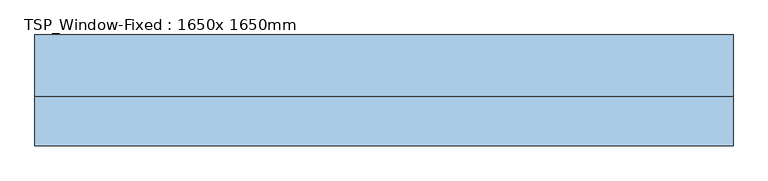
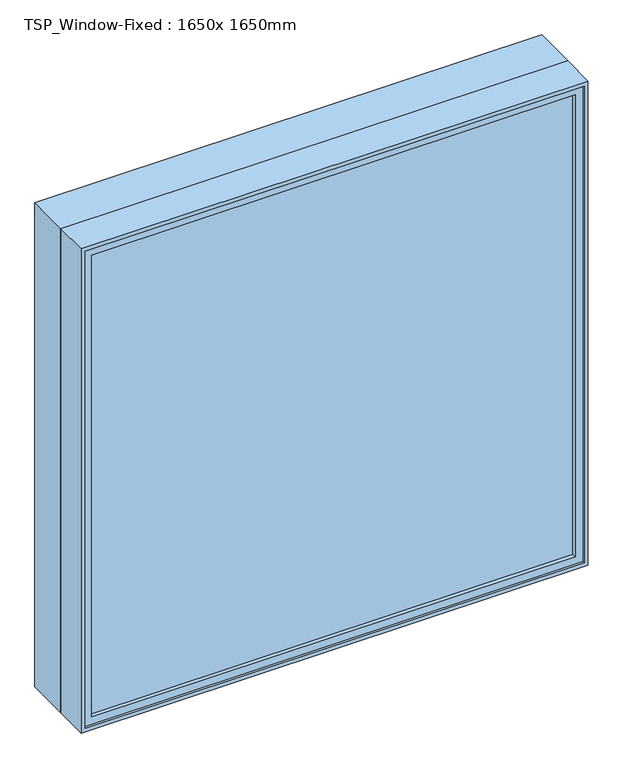
"""IFC4 building model written with IfcOpenShell, lengths in millimetres: window geometry, TSP_Window-Fixed : 1650x 1650mm."""

from ifc_helpers import new_model, si_unit, frame, origin, place, context, project, spatial, polyline, outline, extrude, faceted_brep, source, transform, mapped, element, save


def tsp_window_fixed_1650x_1650mm_face6f7b(model_context):
    return source(origin(), model_context, "Body", "SolidModel", [
        faceted_brep([(817.5, -24.75, 2550.0), (-817.5, -24.75, 2550.0), (-817.5, -139.05, 2550.0), (817.5, -139.05, 2550.0), (-817.5, -24.75, 900.0), (-817.5, -139.05, 900.0), (817.5, -24.75, 900.0), (817.5, -139.05, 900.0), (785.75, -24.75, 2518.25), (-785.75, -24.75, 2518.25), (-785.75, -24.75, 931.75), (785.75, -24.75, 931.75), (-804.8, -139.05, 2537.3), (804.8, -139.05, 2537.3), (804.8, -139.05, 912.7), (-804.8, -139.05, 912.7), (785.75, -88.25, 2518.25), (-785.75, -88.25, 2518.25), (-804.8, -88.25, 2537.3), (804.8, -88.25, 2537.3), (-785.75, -88.25, 931.75), (-804.8, -88.25, 912.7), (785.75, -88.25, 931.75), (804.8, -88.25, 912.7)], [[[0, 1, 2, 3]], [[1, 4, 5, 2]], [[4, 6, 7, 5]], [[1, 0, 6, 4], [8, 9, 10, 11]], [[6, 0, 3, 7]], [[3, 2, 5, 7], [12, 13, 14, 15]], [[16, 17, 9, 8]], [[13, 12, 18, 19]], [[17, 20, 10, 9]], [[12, 15, 21, 18]], [[20, 22, 11, 10]], [[15, 14, 23, 21]], [[22, 16, 8, 11]], [[19, 18, 21, 23], [17, 16, 22, 20]], [[14, 13, 19, 23]]]),
        extrude(outline(polyline([(2550.0, -817.5), (900.0, -817.5), (900.0, 817.5), (2550.0, 817.5), (2550.0, -817.5)]), holes=[polyline([(2537.3, 804.8), (912.7, 804.8), (912.7, -804.8), (2537.3, -804.8), (2537.3, 804.8)])]), frame((0.0, -24.75, 0.0), z_axis=(0.0, 1.0, 0.0), x_axis=(0.0, 0.0, 1.0)), (0.0, 0.0, 1.0), 144.75),
        extrude(outline(polyline([(912.7, -804.8), (912.7, 804.8), (2537.3, 804.8), (2537.3, -804.8), (912.7, -804.8)]), holes=[polyline([(938.1, 779.4), (938.1, -779.4), (2511.9, -779.4), (2511.9, 779.4), (938.1, 779.4)])]), frame((0.0, -132.7, 0.0), z_axis=(0.0, 1.0, 0.0), x_axis=(0.0, 0.0, 1.0)), (0.0, 0.0, 1.0), 44.45),
        extrude(outline(polyline([(779.4, -120.0), (-779.4, -120.0), (-779.4, -113.65), (779.4, -113.65), (779.4, -120.0)])), frame((0.0, 0.0, 938.1), z_axis=(0.0, 0.0, 1.0), x_axis=(1.0, 0.0, 0.0)), (0.0, 0.0, 1.0), 1573.8),
        extrude(outline(polyline([(-779.4, -100.95), (779.4, -100.95), (779.4, -107.3), (-779.4, -107.3), (-779.4, -100.95)])), frame((0.0, 0.0, 938.1), z_axis=(0.0, 0.0, 1.0), x_axis=(1.0, 0.0, 0.0)), (0.0, 0.0, 1.0), 1573.8),
    ])


if __name__ == "__main__":
    model = new_model("IFC4")
    model_context = context("Model", 3, world=origin())
    ifc_project = project(units=[si_unit("LENGTHUNIT", "METRE", prefix="MILLI")], contexts=[model_context])
    site = spatial("IfcSite", under=ifc_project)
    building = spatial("IfcBuilding", under=site)
    placement = place(None, origin())
    tsp_window_fixed_1650x_1650mm_shape = tsp_window_fixed_1650x_1650mm_face6f7b(model_context)
    element("IfcWindow", 1, ObjectType="TSP_Window-Fixed : 1650x 1650mm", at=placement, inside=building, context=model_context, shape_type="MappedRepresentation", body=[
        mapped(tsp_window_fixed_1650x_1650mm_shape, transform((0.0, 0.0, 0.0), x_axis=(1.0, 0.0, 0.0), y_axis=(0.0, 1.0, 0.0), z_axis=(0.0, 0.0, 1.0))),
    ])
    save(model, "model.ifc")

# Revit data of these elements
# Type "TSP_Window-Fixed : 1650x 1650mm"
#   Type Mark = "HS 2412 F154"
#   Fire Rating = "0.5h"
#   Assembly Code = "B2020100"
#   Analytic Construction = "Double glazing - domestic"
#   Window Inset [instance default] = 0 mm
#   Wall Thickness [instance default] = 150 mm
#   Visual Light Transmittance = 0.81
#   Thermal Resistance (R) = 0.319569 (m²·K)/W
#   Solar Heat Gain Coefficient = 0.76
#   Rough Width = 1650 mm
#   Rough Height = 1665 mm
#   Interior Wall Closure [instance default] = 54.75 mm
#   Height = 1650 mm
#   Heat Transfer Coefficient (U) = 3.12929 W/(m²·K)
#   Frame Extension [instance default] = 6.35 mm
#   Exterior Wall Closure [instance default] = 31.75 mm
#   Extension Jamb [instance default] = 54.75 mm
#   Default Sill Height = 900 mm
#   Width = 1635 mm
#   Muntin Visibility = yes
#   Interior Trim Visibility [instance default] = yes
#   Exterior Trim Visibility [instance default] = yes
#   Extension Jamb Visibility [instance default] = yes
#   Interior Trim Material = Wood - Stained
#   Interior Frame Material = Wood - Stained
#   Glass Panel Material = Glass
#   Exterior Trim Material = Clad - White
#   Exterior Frame Material = Clad - White
#   Wall Closure = (empty or 0)
# Element 1 (IfcWindow, "TSP_Window-Fixed : 1650x 1650mm")
#   Wall Thickness = 240 mm
#   Extension Jamb = 144.75 mm
#   Materials on its faces: "Wood - Stained", "Glass", "Clad - White"
# Materials
#   "Wood - Stained": class "Wood", colour RGB 224 178 126, transparency 0, Cost = 0
#   "Glass": class "Glass", colour RGB 0 128 192, transparency 0.9, Description = "Soda Lime Glass", Cost = 0
#   "Clad - White": class "Wood", colour RGB 242 242 238, transparency 0, Cost = 0
